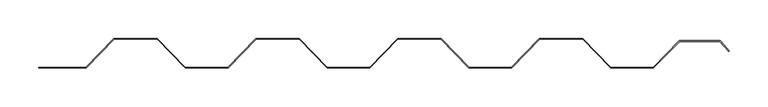
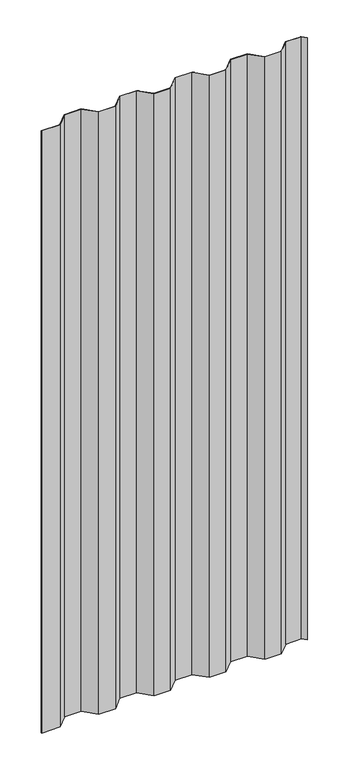
"""IFC4 building model written with IfcOpenShell, lengths in millimetres: proxy geometry, Generic Models 2:Generic Models 2:310765:Generic Models 2:310765 : Generic Models 2:Generic Models 2:310765:16 : Generic Models 2:Generic Models 2:310765:Generic Models 2:310765 : Generic Models 2:Generic Models 2:310765:300385."""

from ifc_helpers import new_model, si_unit, frame, origin, place, context, project, spatial, polyline, outline, extrude, source, transform, mapped, element, save


def generic_models_02d01ef3(model_context):
    return source(origin(), model_context, "Body", "SweptSolid", [
        extrude(outline(polyline([(561244.2659143, -578762.1395469), (561256.1216606, -578775.2476179), (561255.5596888, -578775.8095897), (561243.913577, -578762.9332969), (561192.007223, -578762.9332969), (561158.3752382, -578797.4913841), (561103.1956783, -578797.4913841), (561067.0334867, -578760.1851341), (561011.6583611, -578760.1851341), (560975.4961694, -578797.4913841), (560920.3156783, -578797.4913841), (560884.1534867, -578760.1851341), (560828.7783611, -578760.1851341), (560792.6161694, -578797.4913841), (560737.4356783, -578797.4913841), (560701.2734867, -578760.1851341), (560645.8983611, -578760.1851341), (560609.7361694, -578797.4913841), (560554.5556783, -578797.4913841), (560518.3934867, -578760.1851341), (560463.0183611, -578760.1851341), (560426.8561694, -578797.4913841), (560365.6617239, -578797.4913841), (560365.6617239, -578796.6976341), (560426.5201239, -578796.6976341), (560462.6823155, -578759.3913841), (560518.7295322, -578759.3913841), (560554.8917239, -578796.6976341), (560609.4001239, -578796.6976341), (560645.5623155, -578759.3913841), (560701.6095322, -578759.3913841), (560737.7717239, -578796.6976341), (560792.2801239, -578796.6976341), (560828.4423155, -578759.3913841), (560884.4895322, -578759.3913841), (560920.6517239, -578796.6976341), (560975.1601239, -578796.6976341), (561011.3223155, -578759.3913841), (561067.3695322, -578759.3913841), (561103.5317239, -578796.6976341), (561158.0401239, -578796.6976341), (561191.6721086, -578762.1395469), (561244.2659143, -578762.1395469)])), frame((0.0, 0.0, 4033.8810286), z_axis=(0.0, 0.0, 1.0), x_axis=(1.0, 0.0, 0.0)), (0.0, 0.0, 1.0), 2100.2189714),
    ])


if __name__ == "__main__":
    model = new_model("IFC4")
    model_context = context("Model", 3, world=origin())
    ifc_project = project(units=[si_unit("LENGTHUNIT", "METRE", prefix="MILLI")], contexts=[model_context])
    site = spatial("IfcSite", under=ifc_project)
    building = spatial("IfcBuilding", under=site)
    placement = place(None, origin())
    generic_models_shape = generic_models_02d01ef3(model_context)
    element("IfcBuildingElementProxy", 1, Name="Generic Models 2:Generic Models 2:310765:Generic Models 2:310765 : Generic Models 2:Generic Models 2:310765:16 : Generic Models 2:Generic Models 2:310765:Generic Models 2:310765 : Generic Models 2:Generic Models 2:310765:300385", ObjectType="Generic Models 2:Generic Models 2:310765:Generic Models 2:310765 : Generic Models 2:Generic Models 2:310765:16 : Generic Models 2:Generic Models 2:310765:Generic Models 2:310765 : Generic Models 2:Generic Models 2:310765:300385", at=placement, inside=building, context=model_context, shape_type="MappedRepresentation", body=[
        mapped(generic_models_shape, transform((0.0, 0.0, 0.0), x_axis=(1.0, 0.0, 0.0), y_axis=(0.0, 1.0, 0.0), z_axis=(0.0, 0.0, 1.0))),
    ])
    save(model, "model.ifc")

# Revit data of these elements
# Type "Generic Models 2:Generic Models 2:310765:Generic Models 2:310765 : Generic Models 2:Generic Models 2:310765:16 : Generic Models 2:Generic Models 2:310765:Generic Models 2:310765 : Generic Models 2:Generic Models 2:310765:300385"
#   NameOverride = "Generic Models 2:Generic Models 2:310765:Generic Models 2:310765 : Generic Models 2:Generic Models 2:310765:300385"
#   ObjectTypeOverride = "Generic Models 2:310765 : Generic Models 2:Generic Models 2:310765"
#   Reference = "Generic Models 2"
#   Tag = "300385"
# Element 1 (IfcBuildingElementProxy, "Generic Models 2:Generic Models 2:310765:Generic Models 2:310765 : Generic Models 2:Generic Models 2:310765:16 : Generic Models 2:Generic Models 2:310765:Generic Models 2:310765 : Generic Models 2:Generic Models 2:310765:300385")
#   Materials on its faces: "VERTICAL CORRUGATED METAL PANEL - EXPOSED FASTENERS - (MBCI 7.2 PANEL)"
# Materials
#   "VERTICAL CORRUGATED METAL PANEL - EXPOSED FASTENERS - (MBCI 7.2 PANEL)": class "Generic", colour RGB 120 120 120, transparency 0, Cost = 0
